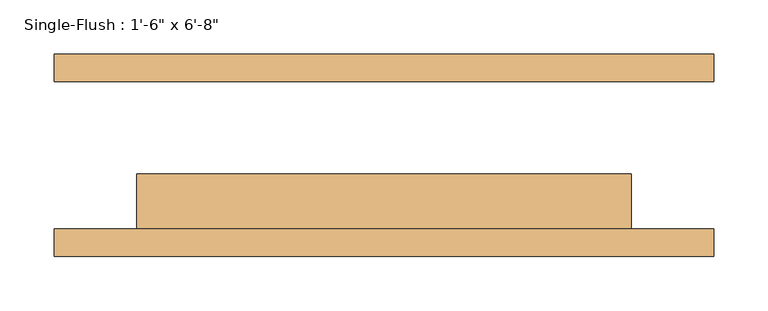
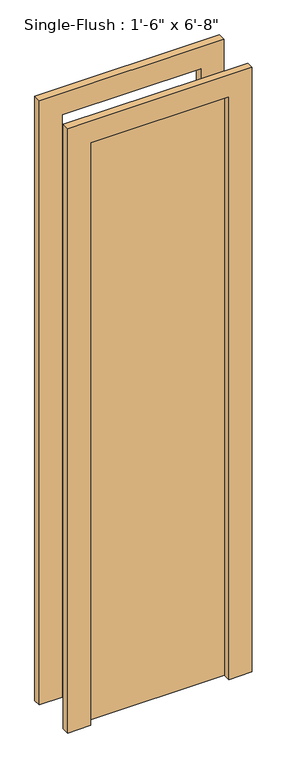
"""IFC4 building model written with IfcOpenShell, lengths in millimetres: door geometry."""

from ifc_helpers import new_model, si_unit, frame, origin, origin_with_axes, place, context, project, spatial, polyline, outline, extrude, source, transform, mapped, element, save


def door_7cdc0a33(model_context):
    return source(origin(), model_context, "Body", "SweptSolid", [
        extrude(outline(polyline([(2108.2, -304.8), (0.0, -304.8), (0.0, -228.6), (2032.0, -228.6), (2032.0, 228.6), (0.0, 228.6), (0.0, 304.8), (2108.2, 304.8), (2108.2, -304.8)])), frame((0.0, -93.6625, 0.0), z_axis=(0.0, 1.0, 0.0), x_axis=(0.0, 0.0, 1.0)), (0.0, 0.0, 1.0), 25.4),
        extrude(outline(polyline([(2108.2, 304.8), (2108.2, -304.8), (0.0, -304.8), (0.0, -228.6), (2032.0, -228.6), (2032.0, 228.6), (0.0, 228.6), (0.0, 304.8), (2108.2, 304.8)])), frame((0.0, 68.2625, 0.0), z_axis=(0.0, 1.0, 0.0), x_axis=(0.0, 0.0, 1.0)), (0.0, 0.0, 1.0), 25.4),
        extrude(outline(polyline([(228.6, -17.4625), (228.6, -68.2625), (-228.6, -68.2625), (-228.6, -17.4625), (228.6, -17.4625)])), origin_with_axes(), (0.0, 0.0, 1.0), 2032.0),
    ])


if __name__ == "__main__":
    model = new_model("IFC4")
    model_context = context("Model", 3, world=origin())
    ifc_project = project(units=[si_unit("LENGTHUNIT", "METRE", prefix="MILLI")], contexts=[model_context])
    site = spatial("IfcSite", under=ifc_project)
    building = spatial("IfcBuilding", under=site)
    placement = place(None, origin())
    door_shape = door_7cdc0a33(model_context)
    element("IfcDoor", 1, ObjectType="Single-Flush : 1'-6\" x 6'-8\"", at=placement, inside=building, context=model_context, shape_type="MappedRepresentation", body=[
        mapped(door_shape, transform((0.0, 0.0, 0.0), x_axis=(1.0, 0.0, 0.0), y_axis=(0.0, 1.0, 0.0), z_axis=(0.0, 0.0, 1.0))),
    ])
    save(model, "model.ifc")

# Revit data of these elements
# Type "Single-Flush : 1'-6\" x 6'-8\""
#   Type Mark = "12"
#   Construction Type Id = "MDOOR"
#   Assembly Code = "C1020"
#   Analytic Construction = "Metal"
#   Thickness = 0' - 2"
#   Heat Transfer Coefficient (U) = 3.7021 W/(m²·K)
#   Height = 6' - 8"
#   Trim Projection Ext = 0' - 1"
#   Trim Projection Int = 0' - 1"
#   Trim Width = 0' - 3"
#   Width = 1' - 6"
#   Door Material = Door - Panel
#   Frame Material = Door - Frame
#   Visual Light Transmittance = 0
#   Solar Heat Gain Coefficient = 0
#   Function = (empty or 0)
#   Wall Closure = (empty or 0)
# Element 1 (IfcDoor, "Single-Flush : 1'-6\" x 6'-8\"")
#   Materials on its faces: "Door - Frame", "Door - Panel"
# Materials
#   "Door - Panel": class "Wood", colour RGB 210 159 95, transparency 0, Cost = 0
#   "Door - Frame": class "Miscellaneous", colour RGB 118 70 51, transparency 0, Cost = 0
